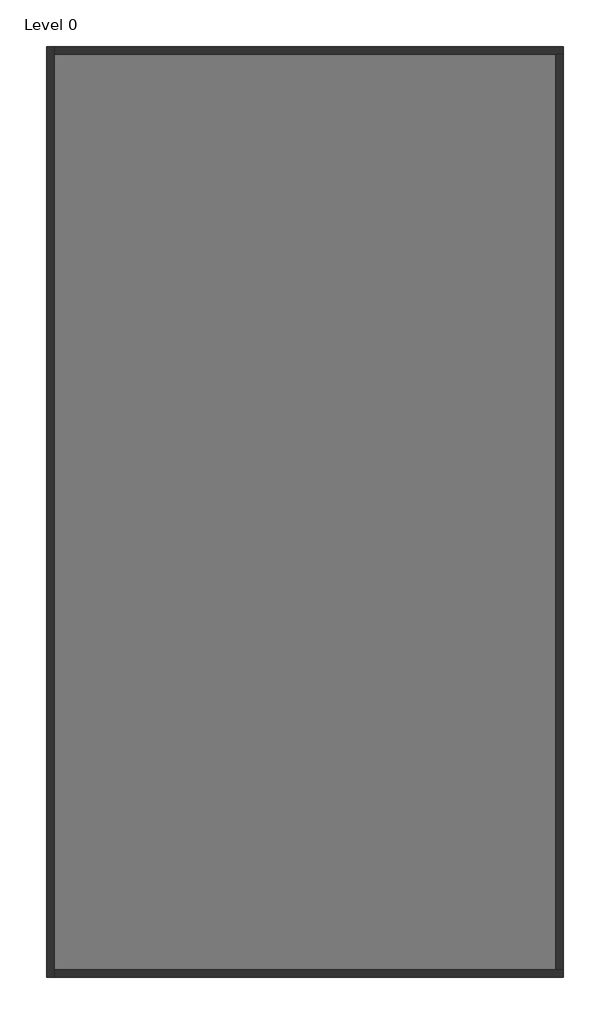
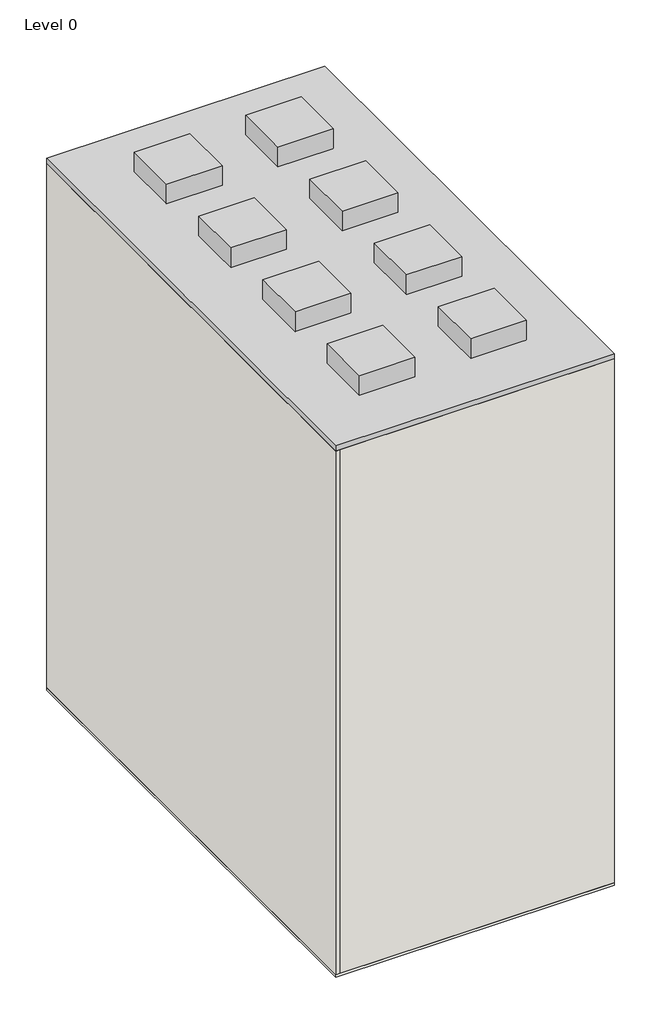
# One storey: 4 walls, 1 proxy, 1 slab.
"""IFC4 building model written with IfcOpenShell, lengths in millimetres."""

from ifc_helpers import new_model, si_unit, frame, origin, origin_with_axes, place, context, project, spatial, polyline, outline, extrude, faceted_brep, element, save

model = new_model("IFC4")

# Units and contexts
model_context = context("Model", 3, world=origin())
ifc_project = project(units=[si_unit("LENGTHUNIT", "METRE", prefix="MILLI")], contexts=[model_context])

# Site, building, storey
site = spatial("IfcSite", under=ifc_project)
building = spatial("IfcBuilding", under=site)
storey = spatial("IfcBuildingStorey", under=building, Name="Level 0", Elevation=100.0)

# Proxy
placement = place(None, origin())
element("IfcBuildingElementProxy", 1, Name="LowUrbanDensityBuilding : LowUrbanDensityBuilding", ObjectType="LowUrbanDensityBuilding : LowUrbanDensityBuilding", at=placement, inside=storey, context=model_context, shape_type="SweptSolid", body=[
    extrude(outline(polyline([(7325.2659446, 3676.2074539), (7325.2659446, -14323.7925461), (-2674.7340554, -14323.7925461), (-2674.7340554, 3676.2074539), (7325.2659446, 3676.2074539)])), origin_with_axes(), (0.0, 0.0, 1.0), 20200.0),
    extrude(outline(polyline([(1325.2659446, 1676.2074539), (1325.2659446, -323.7925461), (-674.7340554, -323.7925461), (-674.7340554, 1676.2074539), (1325.2659446, 1676.2074539)])), frame((0.0, 0.0, 20200.0), z_axis=(0.0, 0.0, 1.0), x_axis=(1.0, 0.0, 0.0)), (0.0, 0.0, 1.0), 749.8),
    extrude(outline(polyline([(5325.2659446, 1676.2074539), (5325.2659446, -323.7925461), (3325.2659446, -323.7925461), (3325.2659446, 1676.2074539), (5325.2659446, 1676.2074539)])), frame((0.0, 0.0, 20200.0), z_axis=(0.0, 0.0, 1.0), x_axis=(1.0, 0.0, 0.0)), (0.0, 0.0, 1.0), 749.8),
    extrude(outline(polyline([(1325.2659446, -2323.7925461), (1325.2659446, -4323.7925461), (-674.7340554, -4323.7925461), (-674.7340554, -2323.7925461), (1325.2659446, -2323.7925461)])), frame((0.0, 0.0, 20200.0), z_axis=(0.0, 0.0, 1.0), x_axis=(1.0, 0.0, 0.0)), (0.0, 0.0, 1.0), 749.8),
    extrude(outline(polyline([(5325.2659446, -2323.7925461), (5325.2659446, -4323.7925461), (3325.2659446, -4323.7925461), (3325.2659446, -2323.7925461), (5325.2659446, -2323.7925461)])), frame((0.0, 0.0, 20200.0), z_axis=(0.0, 0.0, 1.0), x_axis=(1.0, 0.0, 0.0)), (0.0, 0.0, 1.0), 749.8),
    extrude(outline(polyline([(1325.2659446, -6323.7925461), (1325.2659446, -8323.7925461), (-674.7340554, -8323.7925461), (-674.7340554, -6323.7925461), (1325.2659446, -6323.7925461)])), frame((0.0, 0.0, 20200.0), z_axis=(0.0, 0.0, 1.0), x_axis=(1.0, 0.0, 0.0)), (0.0, 0.0, 1.0), 749.8),
    extrude(outline(polyline([(5325.2659446, -6323.7925461), (5325.2659446, -8323.7925461), (3325.2659446, -8323.7925461), (3325.2659446, -6323.7925461), (5325.2659446, -6323.7925461)])), frame((0.0, 0.0, 20200.0), z_axis=(0.0, 0.0, 1.0), x_axis=(1.0, 0.0, 0.0)), (0.0, 0.0, 1.0), 749.8),
    extrude(outline(polyline([(1325.2659446, -10323.7925461), (1325.2659446, -12323.7925461), (-674.7340554, -12323.7925461), (-674.7340554, -10323.7925461), (1325.2659446, -10323.7925461)])), frame((0.0, 0.0, 20200.0), z_axis=(0.0, 0.0, 1.0), x_axis=(1.0, 0.0, 0.0)), (0.0, 0.0, 1.0), 749.8),
    extrude(outline(polyline([(5325.2659446, -10323.7925461), (5325.2659446, -12323.7925461), (3325.2659446, -12323.7925461), (3325.2659446, -10323.7925461), (5325.2659446, -10323.7925461)])), frame((0.0, 0.0, 20200.0), z_axis=(0.0, 0.0, 1.0), x_axis=(1.0, 0.0, 0.0)), (0.0, 0.0, 1.0), 749.8),
])

# Slab
element("IfcSlab", 2, ObjectType="Floor-Concrete_100Con", at=placement, inside=storey, context=model_context, shape_type="SweptSolid", body=[
    extrude(outline(polyline([(7325.2659446, 3676.2074539), (7325.2659446, -14323.7925461), (-2674.7340554, -14323.7925461), (-2674.7340554, 3676.2074539), (7325.2659446, 3676.2074539)])), origin_with_axes(), (0.0, 0.0, 1.0), 100.0),
])

# Walls
element("IfcWall", 3, ObjectType="Wall-Ext_25Rdr-100Blk-19P", at=placement, inside=storey, context=model_context, shape_type="Brep", body=[
    faceted_brep([(-2674.7340554, 3676.2074539, 100.0), (-2674.7340554, -14323.7925461, 100.0), (-2674.7340554, -14323.7925461, 20000.0), (-2674.7340554, 3676.2074539, 20000.0), (-2530.4340554, 3676.2074539, 100.0), (-2530.4340554, 3676.2074539, 20000.0), (-2530.4340554, 3531.9074539, 20000.0), (-2530.4340554, -14179.4925461, 20000.0), (-2530.4340554, -14323.7925461, 20000.0), (-2530.4340554, -14323.7925461, 100.0), (-2530.4340554, -14179.4925461, 100.0), (-2530.4340554, 3531.9074539, 100.0)], [[[0, 1, 2, 3]], [[4, 5, 6, 7, 8, 9, 10, 11]], [[1, 0, 4, 11, 10, 9]], [[3, 2, 8, 7, 6, 5]], [[2, 1, 9, 8]], [[0, 3, 5, 4]]]),
])
element("IfcWall", 4, ObjectType="Wall-Ext_25Rdr-100Blk-19P", at=placement, inside=storey, context=model_context, shape_type="Brep", body=[
    faceted_brep([(-2530.4340554, -14323.7925461, 100.0), (7325.2659446, -14323.7925461, 100.0), (7325.2659446, -14323.7925461, 20000.0), (-2530.4340554, -14323.7925461, 20000.0), (-2530.4340554, -14179.4925461, 100.0), (-2530.4340554, -14179.4925461, 20000.0), (7180.9659446, -14179.4925461, 20000.0), (7325.2659446, -14179.4925461, 20000.0), (7325.2659446, -14179.4925461, 100.0), (7180.9659446, -14179.4925461, 100.0)], [[[0, 1, 2, 3]], [[4, 5, 6, 7, 8, 9]], [[1, 0, 4, 9, 8]], [[3, 2, 7, 6, 5]], [[0, 3, 5, 4]], [[2, 1, 8, 7]]]),
])
element("IfcWall", 5, ObjectType="Wall-Ext_25Rdr-100Blk-19P", at=placement, inside=storey, context=model_context, shape_type="Brep", body=[
    faceted_brep([(7325.2659446, 3676.2074539, 100.0), (-2530.4340554, 3676.2074539, 100.0), (-2530.4340554, 3676.2074539, 20000.0), (7325.2659446, 3676.2074539, 20000.0), (7325.2659446, 3531.9074539, 100.0), (7325.2659446, 3531.9074539, 20000.0), (7180.9659446, 3531.9074539, 20000.0), (-2530.4340554, 3531.9074539, 20000.0), (-2530.4340554, 3531.9074539, 100.0), (7180.9659446, 3531.9074539, 100.0)], [[[0, 1, 2, 3]], [[4, 5, 6, 7, 8, 9]], [[1, 0, 4, 9, 8]], [[3, 2, 7, 6, 5]], [[2, 1, 8, 7]], [[0, 3, 5, 4]]]),
])
element("IfcWall", 6, ObjectType="Wall-Ext_25Rdr-100Blk-19P", at=placement, inside=storey, context=model_context, shape_type="SweptSolid", body=[
    extrude(outline(polyline([(7325.2659446, 3531.9074539), (7325.2659446, -14179.4925461), (7180.9659446, -14179.4925461), (7180.9659446, 3531.9074539), (7325.2659446, 3531.9074539)])), frame((0.0, 0.0, 100.0), z_axis=(0.0, 0.0, 1.0), x_axis=(1.0, 0.0, 0.0)), (0.0, 0.0, 1.0), 19900.0),
])

save(model, "model.ifc")

# Revit data of these elements
# Project information
#   Project Issue Date = "Issue Date"
#   Project Status = "Project Status"
#   Client Name = "Owner"
#   Project Address = "Enter address here"
#   Project Name = "Project Name"
#   Project Number = "Project Number"
# Type "Floor-Concrete_100Con"
#   Keynote = "E60/130"
#   Function = 0
#   Layers, outside or top first: 100 mm "Concrete" (function 1)
# Type "Wall-Ext_25Rdr-100Blk-19P"
#   Keynote = "F10"
#   Layers, outside or top first: 25.3 mm "Render, Beige, Smooth" (function 5); 100 mm "Concrete Masonry Units _Low Density" (function 1); 19 mm "Plaster" (function 5)
# Element 1 (IfcBuildingElementProxy, "LowUrbanDensityBuilding : LowUrbanDensityBuilding")
#   Phase Created = New Construction
#   Materials on its faces: "Default Form"
# Element 2 (IfcSlab, "Floor-Concrete_100Con")
#   Height Offset From Level = 0 mm
#   Phase Created = New Construction
#   Materials on its faces: "Concrete"
# Element 3 (IfcWall, "Wall-Ext_25Rdr-100Blk-19P")
#   Top Offset = 0 mm
#   Base Offset = 0 mm
#   wall height = 19900 mm
#   Phase Created = New Construction
#   Base Constraint = Level 0
#   Top Constraint = Level 5
#   Materials on its faces: "Render, Beige, Smooth", "Default Wall", "Plaster"
# Elements 4, 5, 6 (IfcWall, "Wall-Ext_25Rdr-100Blk-19P")
#   Top Offset = 0 mm
#   Base Offset = 0 mm
#   wall height = 19900 mm
#   Phase Created = New Construction
#   Base Constraint = Level 0
#   Top Constraint = Level 5
#   Materials on its faces: "Default Wall", "Render, Beige, Smooth", "Plaster"
# Materials
#   "Concrete": class "Concrete", colour RGB 120 120 120, transparency 0, Description = "Portland Cement Concrete", Cost = 0
#   "Render, Beige, Smooth": class "Generic", colour RGB 213 198 180, transparency 0, Description = "physical material", Cost = 0
#   "Concrete Masonry Units _Low Density": class "Masonry", colour RGB 181 181 181, transparency 0, Description = "Concrete masonry units", Cost = 0
#   "Plaster": class "Generic", colour RGB 249 249 249, transparency 0, Description = "Plaster", Cost = 0
#   "Default Form": class "Generic", colour RGB 185 189 196, transparency 0.5, Cost = 0
#   "Default Wall": class "Miscellaneous", colour RGB 128 128 128, transparency 0, Comments = "Rendering appearance not upgraded Rendering appearance not upgraded ", Cost = 0
